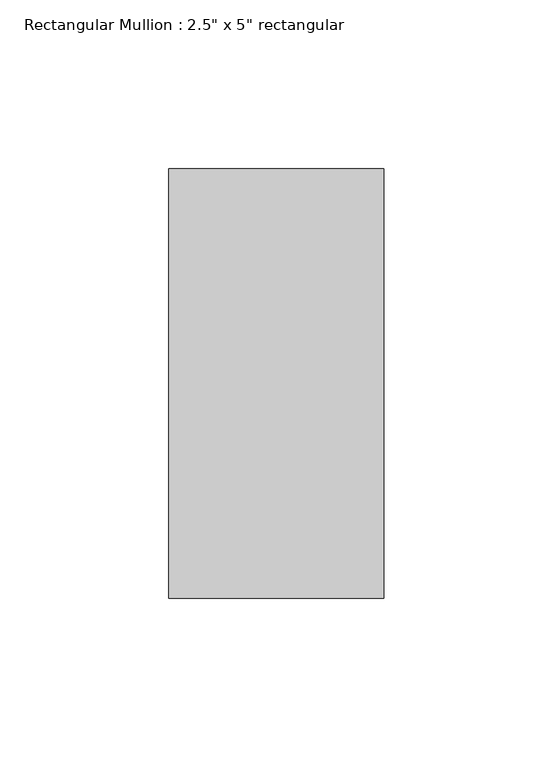
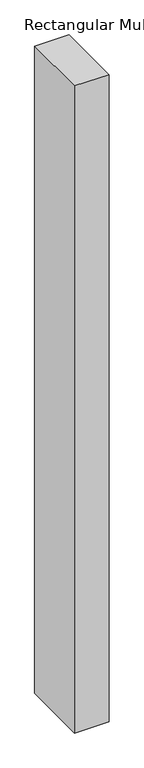
"""IFC4 building model written with IfcOpenShell, lengths in millimetres: member geometry."""

from ifc_helpers import new_model, si_unit, frame, origin, place, context, project, spatial, polyline, outline, extrude, source, transform, mapped, element, save


def member_7bd2cd2c(model_context):
    return source(origin(), model_context, "Body", "SweptSolid", [
        extrude(outline(polyline([(31.75, 63.5), (31.75, -63.5), (-31.75, -63.5), (-31.75, 63.5), (31.75, 63.5)])), frame((0.0, 0.0, -1257.3), z_axis=(0.0, 0.0, 1.0), x_axis=(1.0, 0.0, 0.0)), (0.0, 0.0, 1.0), 1257.3),
    ])


if __name__ == "__main__":
    model = new_model("IFC4")
    model_context = context("Model", 3, world=origin())
    ifc_project = project(units=[si_unit("LENGTHUNIT", "METRE", prefix="MILLI")], contexts=[model_context])
    site = spatial("IfcSite", under=ifc_project)
    building = spatial("IfcBuilding", under=site)
    placement = place(None, origin())
    member_shape = member_7bd2cd2c(model_context)
    element("IfcMember", 1, ObjectType="Rectangular Mullion : 2.5\" x 5\" rectangular", at=placement, inside=building, context=model_context, shape_type="MappedRepresentation", body=[
        mapped(member_shape, transform((0.0, 0.0, 0.0), x_axis=(1.0, 0.0, 0.0), y_axis=(0.0, 1.0, 0.0), z_axis=(0.0, 0.0, 1.0))),
    ])
    save(model, "model.ifc")

# Revit data of these elements
# Type "Rectangular Mullion : 2.5\" x 5\" rectangular"
#   built-in parameter 1007304 = 0.416667 (stored number, unit not read)
#   built-in parameter 1007301 = 0.104167 (stored number, unit not read)
#   built-in parameter 1007300 = 0.104167 (stored number, unit not read)
# Element 1 (IfcMember, "Rectangular Mullion : 2.5\" x 5\" rectangular")
#   Materials on its faces: "Metal - Aluminum"
# Materials
#   "Metal - Aluminum": class "Metal", colour RGB 140 140 140, transparency 0
